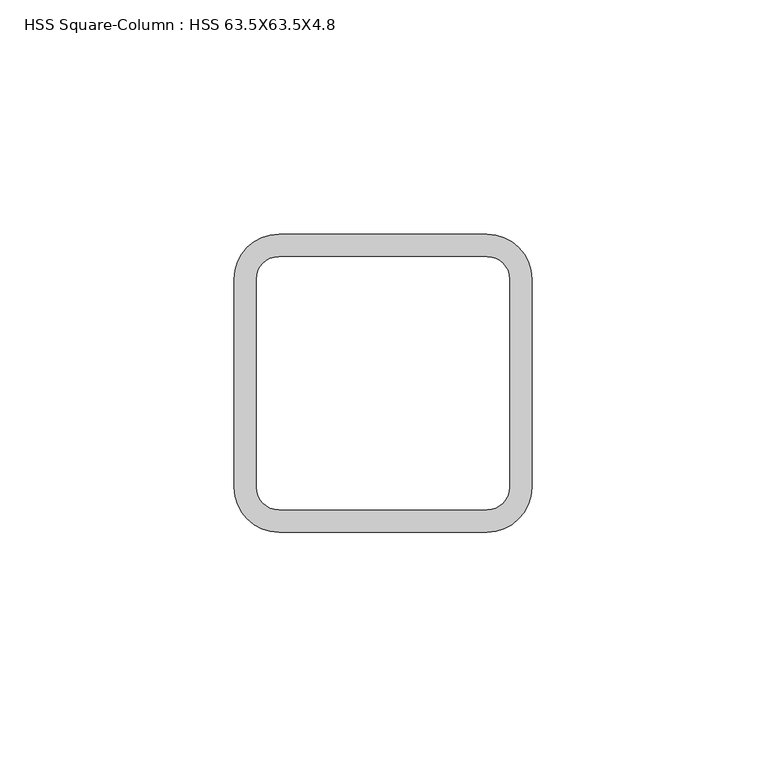
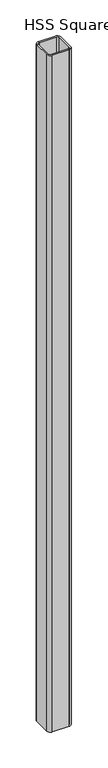
"""IFC4 building model written with IfcOpenShell, lengths in millimetres: column geometry, HSS Square-Column : HSS 63.5X63.5X4.8."""

import ifcopenshell
import ifcopenshell.guid

model = None  # the IFC model being written
_history = None  # IfcOwnerHistory: only IFC2X3 demands one
_inside = {}  # id of a spatial element -> (the spatial element, [elements in it])
_under = {}  # id of a project, library or spatial element -> (it, [spatial elements below it])
_declared = {}  # id of a project -> (the project, [libraries it declares])
_typed = {}  # id of a type object -> (the type object, [elements of that type])
_made_of = {}  # id of a material, layer set ... -> (it, [elements and type objects made of it])


def new_model(schema):
    """Start an empty IFC model of exactly this schema.

    Asked for "IFC4X3", IfcOpenShell would pick the latest addendum, in which some entities
    have other attributes; the version numbers below select the first issue.
    IFC2X3 requires an IfcOwnerHistory on every rooted entity: one is made here for all.
    """
    global model, _history
    if schema == "IFC4X3":
        model = ifcopenshell.file(schema_version=(4, 3, 0, 0))
    else:
        model = ifcopenshell.file(schema=schema)
    _inside.clear()
    _under.clear()
    _declared.clear()
    _typed.clear()
    _made_of.clear()
    _history = None
    if model.schema == "IFC2X3":
        org = make("IfcOrganization", Name="unknown")
        user = make(
            "IfcPersonAndOrganization",
            ThePerson=make("IfcPerson", FamilyName="unknown"),
            TheOrganization=org,
        )
        app = make(
            "IfcApplication",
            ApplicationDeveloper=org,
            Version="unknown",
            ApplicationFullName="unknown",
            ApplicationIdentifier="unknown",
        )
        _history = make(
            "IfcOwnerHistory",
            OwningUser=user,
            OwningApplication=app,
            ChangeAction="ADDED",
            CreationDate=0,
        )
    return model


def make(cls, **values):
    """One entity of the class cls with the attributes given. An attribute that is None is left unset."""
    return model.create_entity(
        cls, **{name: value for name, value in values.items() if value is not None}
    )


def rooted(cls, **values):
    """An entity with a GlobalId (a new one), such as an element, a storey or a relation."""
    return make(cls, GlobalId=ifcopenshell.guid.new(), OwnerHistory=_history, **values)


def si_unit(unit_type, name, prefix=None):
    """IfcSIUnit, for example si_unit("LENGTHUNIT", "METRE", prefix="MILLI")."""
    return make("IfcSIUnit", UnitType=unit_type, Prefix=prefix, Name=name)


def assignment(units):
    """IfcUnitAssignment: the units of a project."""
    return None if units is None else make("IfcUnitAssignment", Units=units)


def point(xyz):
    """IfcCartesianPoint."""
    return None if xyz is None else make("IfcCartesianPoint", Coordinates=xyz)


def direction(xyz):
    """IfcDirection."""
    return None if xyz is None else make("IfcDirection", DirectionRatios=xyz)


def frame(location, z_axis=None, x_axis=None):
    """IfcAxis2Placement3D, a coordinate frame: its origin and axes. An axis left out is left unset."""
    return make(
        "IfcAxis2Placement3D",
        Location=point(location),
        Axis=direction(z_axis),
        RefDirection=direction(x_axis),
    )


def frame_2d(location, x_axis=None):
    """IfcAxis2Placement2D, a coordinate frame in the plane: its origin and x axis."""
    return make(
        "IfcAxis2Placement2D", Location=point(location), RefDirection=direction(x_axis)
    )


def origin():
    """The frame at (0, 0, 0) with its axes left unset."""
    return frame((0.0, 0.0, 0.0))


def place(relative_to, where):
    """IfcLocalPlacement: puts the frame where relative to a parent placement (None: the world)."""
    return make(
        "IfcLocalPlacement", PlacementRelTo=relative_to, RelativePlacement=where
    )


def context(
    kind, dimensions, precision=None, world=None, true_north=None, identifier=None
):
    """IfcGeometricRepresentationContext, for example the 3D "Model" context."""
    return make(
        "IfcGeometricRepresentationContext",
        ContextIdentifier=identifier,
        ContextType=kind,
        CoordinateSpaceDimension=dimensions,
        Precision=precision,
        WorldCoordinateSystem=world,
        TrueNorth=true_north,
    )


def project(units=None, contexts=None):
    """IfcProject with its units and contexts."""
    return rooted(
        "IfcProject",
        Name="project",
        RepresentationContexts=contexts,
        UnitsInContext=assignment(units),
    )


def spatial(cls, under=None, at=None, **own):
    """A site, building, storey or space (cls), placed at a placement, below another one or the project."""
    s = rooted(cls, ObjectPlacement=at, **own)
    if under is not None:
        _under.setdefault(under.id(), (under, []))[1].append(s)
    return s


def polyline(points):
    """IfcPolyline through the points."""
    return make("IfcPolyline", Points=[point(p) for p in points])


def circle_curve(where, radius):
    """IfcCircle in the frame where."""
    return make("IfcCircle", Position=where, Radius=radius)


def trimmed(basis, trim1, trim2, sense, master):
    """IfcTrimmedCurve: the piece of a basis curve between two trims."""
    return make(
        "IfcTrimmedCurve",
        BasisCurve=basis,
        Trim1=trim1,
        Trim2=trim2,
        SenseAgreement=sense,
        MasterRepresentation=master,
    )


def segment(curve, same_sense, transition):
    """IfcCompositeCurveSegment."""
    return make(
        "IfcCompositeCurveSegment",
        Transition=transition,
        SameSense=same_sense,
        ParentCurve=curve,
    )


def composite_curve(segments, self_intersect=None):
    """IfcCompositeCurve: segments joined end to end."""
    return make("IfcCompositeCurve", Segments=segments, SelfIntersect=self_intersect)


def outline(outer, holes=None, kind="AREA"):
    """IfcArbitraryClosedProfileDef: a profile drawn as a closed curve; with holes, ...WithVoids."""
    if holes is None:
        return make("IfcArbitraryClosedProfileDef", ProfileType=kind, OuterCurve=outer)
    return make(
        "IfcArbitraryProfileDefWithVoids",
        ProfileType=kind,
        OuterCurve=outer,
        InnerCurves=holes,
    )


def extrude(swept, where, along, depth):
    """IfcExtrudedAreaSolid: the profile swept, set in the frame where, extruded along a direction by depth."""
    return make(
        "IfcExtrudedAreaSolid",
        SweptArea=swept,
        Position=where,
        ExtrudedDirection=direction(along),
        Depth=depth,
    )


def shape(context_of_items, identifier, shape_type, items):
    """IfcShapeRepresentation: the items that make up one representation, for example the "Body"."""
    return make(
        "IfcShapeRepresentation",
        ContextOfItems=context_of_items,
        RepresentationIdentifier=identifier,
        RepresentationType=shape_type,
        Items=items,
    )


def source(mapping_origin, context_of_items, identifier, shape_type, items):
    """IfcRepresentationMap: a shape defined once, which mapped items show again and again."""
    return make(
        "IfcRepresentationMap",
        MappingOrigin=mapping_origin,
        MappedRepresentation=shape(context_of_items, identifier, shape_type, items),
    )


def transform(
    local_origin,
    x_axis=None,
    y_axis=None,
    z_axis=None,
    scale=None,
    scale2=None,
    scale3=None,
    uniform=True,
):
    """IfcCartesianTransformationOperator3D, or its non-uniform kind. x_axis, y_axis, z_axis: its Axis1, 2, 3."""
    if uniform:
        return make(
            "IfcCartesianTransformationOperator3D",
            Axis1=direction(x_axis),
            Axis2=direction(y_axis),
            LocalOrigin=point(local_origin),
            Scale=scale,
            Axis3=direction(z_axis),
        )
    return make(
        "IfcCartesianTransformationOperator3DnonUniform",
        Axis1=direction(x_axis),
        Axis2=direction(y_axis),
        LocalOrigin=point(local_origin),
        Scale=scale,
        Axis3=direction(z_axis),
        Scale2=scale2,
        Scale3=scale3,
    )


def mapped(mapping_source, mapping_target):
    """IfcMappedItem: shows the shape of a source again, moved by a transform."""
    return make(
        "IfcMappedItem", MappingSource=mapping_source, MappingTarget=mapping_target
    )


def made_of(thing, what):
    """Note that an element or type object is made of a material, layer set ...; save() writes the relation."""
    if what is not None:
        _made_of.setdefault(what.id(), (what, []))[1].append(thing)
    return thing


def element(
    cls,
    number,
    at=None,
    inside=None,
    cuts=None,
    type_object=None,
    material=None,
    context=None,
    identifier="Body",
    shape_type=None,
    held_by="IfcProductDefinitionShape",
    body=None,
    shapes=None,
    **own,
):
    """One element of the class cls, such as IfcWall. Its Tag is "e" and its number.

    at: its placement. inside: the storey or other place that contains it. cuts: it is an
    opening in that element (IfcRelVoidsElement). A single representation is given by context,
    identifier, shape_type and body (its items); several are given by shapes. held_by: the class
    of the entity that holds the representations. save() writes the other relations.
    """
    e = rooted(cls, Tag="e%d" % number, ObjectPlacement=at, **own)
    if body is not None:
        shapes = [shape(context, identifier, shape_type, body)]
    if shapes is not None:
        e.Representation = make(held_by, Representations=shapes)
    if inside is not None:
        _inside.setdefault(inside.id(), (inside, []))[1].append(e)
    if cuts is not None:
        rooted(
            "IfcRelVoidsElement", RelatingBuildingElement=cuts, RelatedOpeningElement=e
        )
    if type_object is not None:
        _typed.setdefault(type_object.id(), (type_object, []))[1].append(e)
    return made_of(e, material)


def aggregate(whole, parts):
    """IfcRelAggregates: a whole, such as a stair, and the parts it consists of."""
    return rooted("IfcRelAggregates", RelatingObject=whole, RelatedObjects=parts)


def save(model, path):
    """Write the relations noted so far, then the file.

    IfcRelAggregates (storeys below a building ...), IfcRelContainedInSpatialStructure (elements
    in a storey), IfcRelDefinesByType, IfcRelAssociatesMaterial and IfcRelDeclares: one each for
    every whole, place, type object, material and project.
    """
    for whole, parts in _under.values():
        aggregate(whole, parts)
    for where, things in _inside.values():
        rooted(
            "IfcRelContainedInSpatialStructure",
            RelatedElements=things,
            RelatingStructure=where,
        )
    for kind, things in _typed.values():
        rooted("IfcRelDefinesByType", RelatedObjects=things, RelatingType=kind)
    for what, things in _made_of.values():
        rooted("IfcRelAssociatesMaterial", RelatedObjects=things, RelatingMaterial=what)
    for by, libraries in _declared.values():
        rooted("IfcRelDeclares", RelatingContext=by, RelatedDefinitions=libraries)
    model.write(path)


def hss_square_column_hss_63_5x63_5x4_8_25e297bd(model_context):
    return source(origin(), model_context, "Body", "SweptSolid", [
        extrude(outline(composite_curve([segment(trimmed(circle_curve(frame_2d((22.225, 22.225)), 9.525), [point((22.225, 31.75))], [point((31.75, 22.225))], False, "CARTESIAN"), True, "CONTINUOUS"), segment(polyline([(31.75, 22.225), (31.75, -22.225)]), True, "CONTINUOUS"), segment(trimmed(circle_curve(frame_2d((22.225, -22.225)), 9.525), [point((31.75, -22.225))], [point((22.225, -31.75))], False, "CARTESIAN"), True, "CONTINUOUS"), segment(polyline([(22.225, -31.75), (-22.225, -31.75)]), True, "CONTINUOUS"), segment(trimmed(circle_curve(frame_2d((-22.225, -22.225)), 9.525), [point((-22.225, -31.75))], [point((-31.75, -22.225))], False, "CARTESIAN"), True, "CONTINUOUS"), segment(polyline([(-31.75, -22.225), (-31.75, 22.225)]), True, "CONTINUOUS"), segment(trimmed(circle_curve(frame_2d((-22.225, 22.225)), 9.525), [point((-31.75, 22.225))], [point((-22.225, 31.75))], False, "CARTESIAN"), True, "CONTINUOUS"), segment(polyline([(-22.225, 31.75), (22.225, 31.75)]), True, "CONTINUOUS")], self_intersect=False), holes=[composite_curve([segment(polyline([(22.225, 26.9875), (-22.225, 26.9875)]), True, "CONTINUOUS"), segment(trimmed(circle_curve(frame_2d((-22.225, 22.225)), 4.7625), [point((-22.225, 26.9875))], [point((-26.9875, 22.225))], True, "CARTESIAN"), True, "CONTINUOUS"), segment(polyline([(-26.9875, 22.225), (-26.9875, -22.225)]), True, "CONTINUOUS"), segment(trimmed(circle_curve(frame_2d((-22.225, -22.225)), 4.7625), [point((-26.9875, -22.225))], [point((-22.225, -26.9875))], True, "CARTESIAN"), True, "CONTINUOUS"), segment(polyline([(-22.225, -26.9875), (22.225, -26.9875)]), True, "CONTINUOUS"), segment(trimmed(circle_curve(frame_2d((22.225, -22.225)), 4.7625), [point((22.225, -26.9875))], [point((26.9875, -22.225))], True, "CARTESIAN"), True, "CONTINUOUS"), segment(polyline([(26.9875, -22.225), (26.9875, 22.225)]), True, "CONTINUOUS"), segment(trimmed(circle_curve(frame_2d((22.225, 22.225)), 4.7625), [point((26.9875, 22.225))], [point((22.225, 26.9875))], True, "CARTESIAN"), True, "CONTINUOUS")], self_intersect=False)]), frame((0.0, 0.0, 3220.0), z_axis=(0.0, 0.0, 1.0), x_axis=(1.0, 0.0, 0.0)), (0.0, 0.0, 1.0), 1900.0),
    ])


if __name__ == "__main__":
    model = new_model("IFC4")
    model_context = context("Model", 3, world=origin())
    ifc_project = project(units=[si_unit("LENGTHUNIT", "METRE", prefix="MILLI")], contexts=[model_context])
    site = spatial("IfcSite", under=ifc_project)
    building = spatial("IfcBuilding", under=site)
    placement = place(None, origin())
    hss_square_column_hss_63_5x63_5x4_8_shape = hss_square_column_hss_63_5x63_5x4_8_25e297bd(model_context)
    element("IfcColumn", 1, ObjectType="HSS Square-Column : HSS 63.5X63.5X4.8", at=placement, inside=building, context=model_context, shape_type="MappedRepresentation", body=[
        mapped(hss_square_column_hss_63_5x63_5x4_8_shape, transform((0.0, 0.0, 0.0), x_axis=(1.0, 0.0, 0.0), y_axis=(0.0, 1.0, 0.0), z_axis=(0.0, 0.0, 1.0))),
    ])
    save(model, "model.ifc")

# Revit data of these elements
# Type "HSS Square-Column : HSS 63.5X63.5X4.8"
#   Section Name Key = "HSS 2 1/2X2 1/2X3/16"
#   Assembly Code = "B10"
#   Width = 6.35 cm
#   Wall Nominal Thickness = 0.4763 cm
#   Wall Design Thickness = 0.442 cm
#   Torsional Moment of Inertia = 93.6521 cm⁴
#   Torsional Modulus = 30.4799 cm³
#   Section Area = 9.93546 cm²
#   Plastic Modulus weak axis = 21.6309 cm³
#   Plastic Modulus strong axis = 21.6309 cm³
#   Outer Fillet = 0.9525 cm
#   Nominal Weight = 8.31884 kgf/m
#   Moment of Inertia weak axis = 56.1912 cm⁴
#   Moment of Inertia strong axis = 56.1912 cm⁴
#   Inner Fillet = 0.4763 cm
#   Height = 6.35 cm
#   Elastic Modulus weak axis = 17.698 cm³
#   Elastic Modulus strong axis = 17.698 cm³
#   Centroid Vertical = 3.175 cm
#   Centroid Horizontal = 3.175 cm
#   Structural Material [instance default] = Steel ASTM A500, Grade B, Rectangular and Square
#   Principal Axes Angle = 0
# Element 1 (IfcColumn, "HSS Square-Column : HSS 63.5X63.5X4.8")
#   Structural Material = none
# Materials
#   "Steel ASTM A500, Grade B, Rectangular and Square": class "Metal", colour RGB 199 199 199, transparency 0, Description = "Carbon steel", Cost = 0
